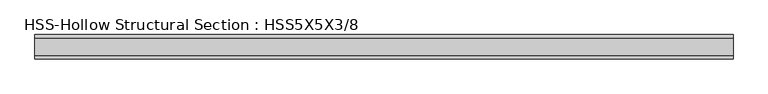
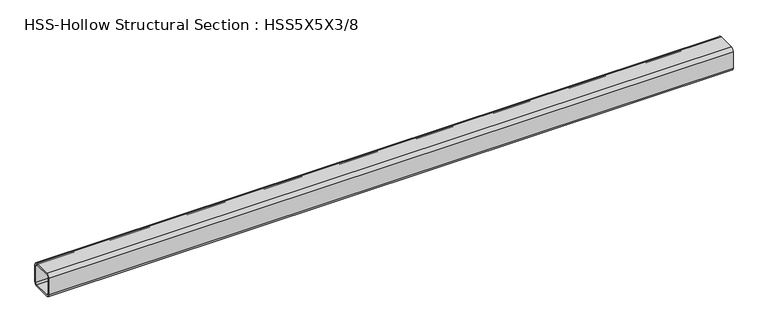
"""IFC4 building model written with IfcOpenShell, lengths in millimetres: member geometry, HSS-Hollow Structural Section : HSS5X5X3/8."""

from ifc_helpers import new_model, si_unit, point, frame, frame_2d, origin, place, context, project, spatial, polyline, circle_curve, trimmed, segment, composite_curve, outline, extrude, source, transform, mapped, element, save


def hss_hollow_structural_section_hss5x5x3_8_70fbec79(model_context):
    return source(origin(), model_context, "Body", "SweptSolid", [
        extrude(outline(composite_curve([segment(polyline([(63.5, 45.7708), (63.5, -45.7708)]), True, "CONTINUOUS"), segment(trimmed(circle_curve(frame_2d((45.7708, -45.7708)), 17.7292), [point((63.5, -45.7708))], [point((45.7708, -63.5))], False, "CARTESIAN"), True, "CONTINUOUS"), segment(polyline([(45.7708, -63.5), (-45.7708, -63.5)]), True, "CONTINUOUS"), segment(trimmed(circle_curve(frame_2d((-45.7708, -45.7708)), 17.7292), [point((-45.7708, -63.5))], [point((-63.5, -45.7708))], False, "CARTESIAN"), True, "CONTINUOUS"), segment(polyline([(-63.5, -45.7708), (-63.5, 45.7708)]), True, "CONTINUOUS"), segment(trimmed(circle_curve(frame_2d((-45.7708, 45.7708)), 17.7292), [point((-63.5, 45.7708))], [point((-45.7708, 63.5))], False, "CARTESIAN"), True, "CONTINUOUS"), segment(polyline([(-45.7708, 63.5), (45.7708, 63.5)]), True, "CONTINUOUS"), segment(trimmed(circle_curve(frame_2d((45.7708, 45.7708)), 17.7292), [point((45.7708, 63.5))], [point((63.5, 45.7708))], False, "CARTESIAN"), True, "CONTINUOUS")], self_intersect=False), holes=[composite_curve([segment(trimmed(circle_curve(frame_2d((-45.7708, 45.7708)), 8.8646), [point((-45.7708, 54.6354))], [point((-54.6354, 45.7708))], True, "CARTESIAN"), True, "CONTINUOUS"), segment(polyline([(-54.6354, 45.7708), (-54.6354, -45.7708)]), True, "CONTINUOUS"), segment(trimmed(circle_curve(frame_2d((-45.7708, -45.7708)), 8.8646), [point((-54.6354, -45.7708))], [point((-45.7708, -54.6354))], True, "CARTESIAN"), True, "CONTINUOUS"), segment(polyline([(-45.7708, -54.6354), (45.7708, -54.6354)]), True, "CONTINUOUS"), segment(trimmed(circle_curve(frame_2d((45.7708, -45.7708)), 8.8646), [point((45.7708, -54.6354))], [point((54.6354, -45.7708))], True, "CARTESIAN"), True, "CONTINUOUS"), segment(polyline([(54.6354, -45.7708), (54.6354, 45.7708)]), True, "CONTINUOUS"), segment(trimmed(circle_curve(frame_2d((45.7708, 45.7708)), 8.8646), [point((54.6354, 45.7708))], [point((45.7708, 54.6354))], True, "CARTESIAN"), True, "CONTINUOUS"), segment(polyline([(45.7708, 54.6354), (-45.7708, 54.6354)]), True, "CONTINUOUS")], self_intersect=False)]), frame((-1810.5215182, 0.0, 0.0), z_axis=(1.0, 0.0, 0.0), x_axis=(0.0, 1.0, 0.0)), (0.0, 0.0, 1.0), 3621.0430365),
    ])


if __name__ == "__main__":
    model = new_model("IFC4")
    model_context = context("Model", 3, world=origin())
    ifc_project = project(units=[si_unit("LENGTHUNIT", "METRE", prefix="MILLI")], contexts=[model_context])
    site = spatial("IfcSite", under=ifc_project)
    building = spatial("IfcBuilding", under=site)
    placement = place(None, origin())
    hss_hollow_structural_section_hss5x5x3_8_shape = hss_hollow_structural_section_hss5x5x3_8_70fbec79(model_context)
    element("IfcMember", 1, ObjectType="HSS-Hollow Structural Section : HSS5X5X3/8", at=placement, inside=building, context=model_context, shape_type="MappedRepresentation", body=[
        mapped(hss_hollow_structural_section_hss5x5x3_8_shape, transform((0.0, 0.0, 0.0), x_axis=(1.0, 0.0, 0.0), y_axis=(0.0, 1.0, 0.0), z_axis=(0.0, 0.0, 1.0))),
    ])
    save(model, "model.ifc")

# Revit data of these elements
# Type "HSS-Hollow Structural Section : HSS5X5X3/8"
#   Assembly Code = "B10"
#   Shape = "Square"
#   W = 22.3
#   Ht = 0' - 5"
#   Length [instance default] = 5' - 0"
#   b = 0' - 5"
#   kr = 0' - 0.698"
#   t = 0' - 0.349"
#   A = 0.0429167 SF
#   Structural Material [instance default] = Steel ASTM A500, Grade B, Rectangular and Square
# Element 1 (IfcMember, "HSS-Hollow Structural Section : HSS5X5X3/8")
#   Materials on its faces: "Steel ASTM A500, Grade B, Rectangular and Square"
# Materials
#   "Steel ASTM A500, Grade B, Rectangular and Square": class "Metal", colour RGB 199 199 199, transparency 0, Description = "Carbon steel", Cost = 0
